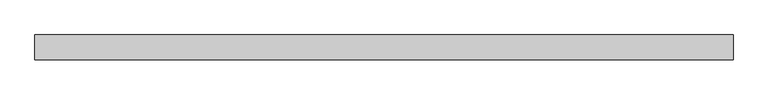
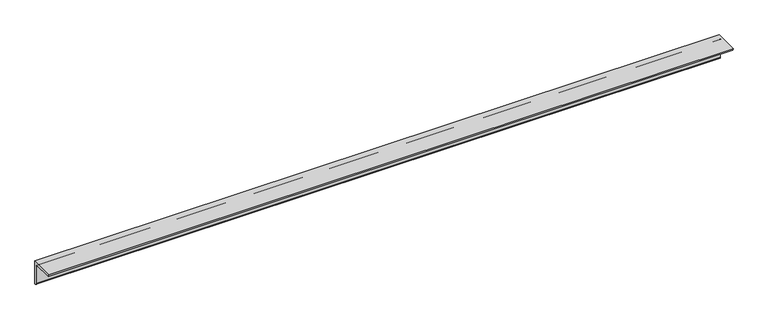
"""IFC4 building model written with IfcOpenShell, lengths in millimetres: member geometry, 0912_Steel Framing_L-KSD3502 : H_SB_AR_S03_L-130x130x12_HBR3."""

from ifc_helpers import new_model, si_unit, point, frame, frame_2d, origin, place, context, project, spatial, polyline, circle_curve, trimmed, segment, composite_curve, outline, extrude, source, transform, mapped, element, save


def member_c6234845(model_context):
    return source(origin(), model_context, "Body", "SweptSolid", [
        extrude(outline(composite_curve([segment(polyline([(36.4, 36.4), (36.4, -93.6)]), True, "CONTINUOUS"), segment(trimmed(circle_curve(frame_2d((36.4, -81.6)), 12.0), [point((36.4, -93.6))], [point((24.4, -81.6))], False, "CARTESIAN"), True, "CONTINUOUS"), segment(polyline([(24.4, -81.6), (24.4, 12.4)]), True, "CONTINUOUS"), segment(trimmed(circle_curve(frame_2d((12.4, 12.4)), 12.0), [point((24.4, 12.4))], [point((12.4, 24.4))], True, "CARTESIAN"), True, "CONTINUOUS"), segment(polyline([(12.4, 24.4), (-81.6, 24.4)]), True, "CONTINUOUS"), segment(trimmed(circle_curve(frame_2d((-81.6, 36.4)), 12.0), [point((-81.6, 24.4))], [point((-93.6, 36.4))], False, "CARTESIAN"), True, "CONTINUOUS"), segment(polyline([(-93.6, 36.4), (36.4, 36.4)]), True, "CONTINUOUS")], self_intersect=False)), frame((-1792.1825023, 0.0, 0.0), z_axis=(1.0, 0.0, 0.0), x_axis=(0.0, 1.0, 0.0)), (0.0, 0.0, 1.0), 3659.8690046),
    ])


if __name__ == "__main__":
    model = new_model("IFC4")
    model_context = context("Model", 3, world=origin())
    ifc_project = project(units=[si_unit("LENGTHUNIT", "METRE", prefix="MILLI")], contexts=[model_context])
    site = spatial("IfcSite", under=ifc_project)
    building = spatial("IfcBuilding", under=site)
    placement = place(None, origin())
    member_shape = member_c6234845(model_context)
    element("IfcMember", 1, ObjectType="0912_Steel Framing_L-KSD3502 : H_SB_AR_S03_L-130x130x12_HBR3", at=placement, inside=building, context=model_context, shape_type="MappedRepresentation", body=[
        mapped(member_shape, transform((0.0, 0.0, 0.0), x_axis=(1.0, 0.0, 0.0), y_axis=(0.0, 1.0, 0.0), z_axis=(0.0, 0.0, 1.0))),
    ])
    save(model, "model.ifc")

# Revit data of these elements
# Type "0912_Steel Framing_L-KSD3502 : H_SB_AR_S03_L-130x130x12_HBR3"
#   k = 25 mm
#   Perimeter = 0.52 m²/m
#   Nominal Weight = 23.40 kgf/m
#   Length [instance default] = 1000 mm
#   b = 130 mm
#   d = 130 mm
#   t = 12 mm
#   x = 36.4 mm
#   y = 36.4 mm
#   A = 2976.00 m²
#   Structural Material [instance default] = Steel, 45-345
# Element 1 (IfcMember, "0912_Steel Framing_L-KSD3502 : H_SB_AR_S03_L-130x130x12_HBR3")
#   Structural Material = Steel ASTM A36
#   Materials on its faces: "Steel ASTM A36"
# Materials
#   "Steel, 45-345": class "Metal", colour RGB 189 187 185, transparency 0, Description = "Steel 345 MPa", Cost = 0
#   "Steel ASTM A36": class "Metal", colour RGB 199 199 199, transparency 0, Description = "Structural steel, ASTM A36 Grade B, mill finish", Cost = 0
